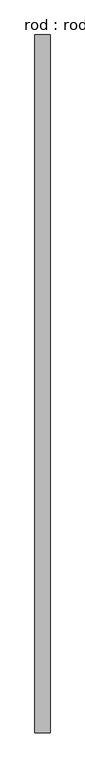
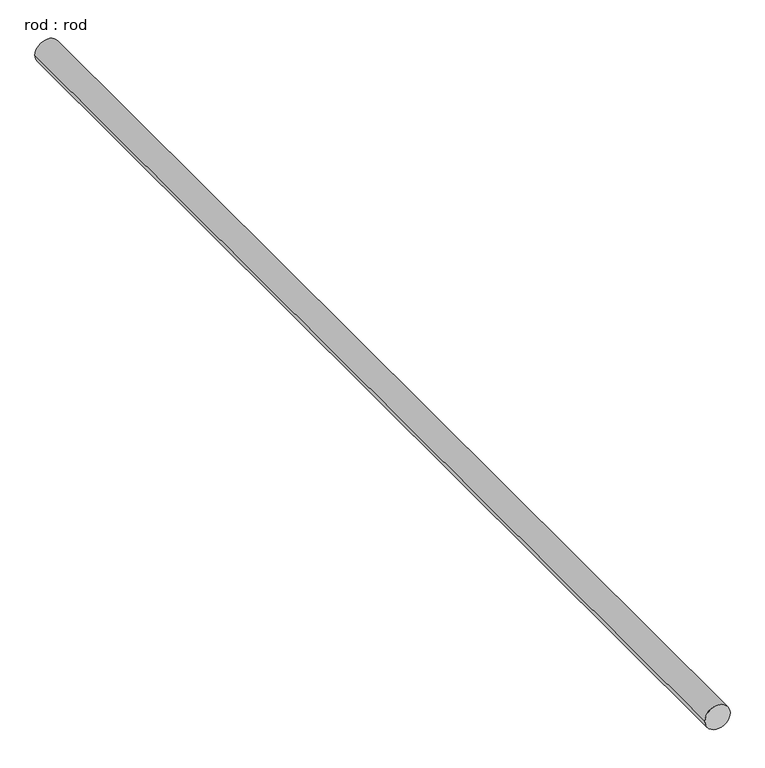
"""IFC4 building model written with IfcOpenShell, lengths in millimetres: proxy geometry, rod : rod."""

import ifcopenshell
import ifcopenshell.guid

model = None  # the IFC model being written
_history = None  # IfcOwnerHistory: only IFC2X3 demands one
_inside = {}  # id of a spatial element -> (the spatial element, [elements in it])
_under = {}  # id of a project, library or spatial element -> (it, [spatial elements below it])
_declared = {}  # id of a project -> (the project, [libraries it declares])
_typed = {}  # id of a type object -> (the type object, [elements of that type])
_made_of = {}  # id of a material, layer set ... -> (it, [elements and type objects made of it])


def new_model(schema):
    """Start an empty IFC model of exactly this schema.

    Asked for "IFC4X3", IfcOpenShell would pick the latest addendum, in which some entities
    have other attributes; the version numbers below select the first issue.
    IFC2X3 requires an IfcOwnerHistory on every rooted entity: one is made here for all.
    """
    global model, _history
    if schema == "IFC4X3":
        model = ifcopenshell.file(schema_version=(4, 3, 0, 0))
    else:
        model = ifcopenshell.file(schema=schema)
    _inside.clear()
    _under.clear()
    _declared.clear()
    _typed.clear()
    _made_of.clear()
    _history = None
    if model.schema == "IFC2X3":
        org = make("IfcOrganization", Name="unknown")
        user = make(
            "IfcPersonAndOrganization",
            ThePerson=make("IfcPerson", FamilyName="unknown"),
            TheOrganization=org,
        )
        app = make(
            "IfcApplication",
            ApplicationDeveloper=org,
            Version="unknown",
            ApplicationFullName="unknown",
            ApplicationIdentifier="unknown",
        )
        _history = make(
            "IfcOwnerHistory",
            OwningUser=user,
            OwningApplication=app,
            ChangeAction="ADDED",
            CreationDate=0,
        )
    return model


def make(cls, **values):
    """One entity of the class cls with the attributes given. An attribute that is None is left unset."""
    return model.create_entity(
        cls, **{name: value for name, value in values.items() if value is not None}
    )


def rooted(cls, **values):
    """An entity with a GlobalId (a new one), such as an element, a storey or a relation."""
    return make(cls, GlobalId=ifcopenshell.guid.new(), OwnerHistory=_history, **values)


def si_unit(unit_type, name, prefix=None):
    """IfcSIUnit, for example si_unit("LENGTHUNIT", "METRE", prefix="MILLI")."""
    return make("IfcSIUnit", UnitType=unit_type, Prefix=prefix, Name=name)


def assignment(units):
    """IfcUnitAssignment: the units of a project."""
    return None if units is None else make("IfcUnitAssignment", Units=units)


def point(xyz):
    """IfcCartesianPoint."""
    return None if xyz is None else make("IfcCartesianPoint", Coordinates=xyz)


def direction(xyz):
    """IfcDirection."""
    return None if xyz is None else make("IfcDirection", DirectionRatios=xyz)


def frame(location, z_axis=None, x_axis=None):
    """IfcAxis2Placement3D, a coordinate frame: its origin and axes. An axis left out is left unset."""
    return make(
        "IfcAxis2Placement3D",
        Location=point(location),
        Axis=direction(z_axis),
        RefDirection=direction(x_axis),
    )


def frame_2d(location, x_axis=None):
    """IfcAxis2Placement2D, a coordinate frame in the plane: its origin and x axis."""
    return make(
        "IfcAxis2Placement2D", Location=point(location), RefDirection=direction(x_axis)
    )


def origin():
    """The frame at (0, 0, 0) with its axes left unset."""
    return frame((0.0, 0.0, 0.0))


def place(relative_to, where):
    """IfcLocalPlacement: puts the frame where relative to a parent placement (None: the world)."""
    return make(
        "IfcLocalPlacement", PlacementRelTo=relative_to, RelativePlacement=where
    )


def context(
    kind, dimensions, precision=None, world=None, true_north=None, identifier=None
):
    """IfcGeometricRepresentationContext, for example the 3D "Model" context."""
    return make(
        "IfcGeometricRepresentationContext",
        ContextIdentifier=identifier,
        ContextType=kind,
        CoordinateSpaceDimension=dimensions,
        Precision=precision,
        WorldCoordinateSystem=world,
        TrueNorth=true_north,
    )


def project(units=None, contexts=None):
    """IfcProject with its units and contexts."""
    return rooted(
        "IfcProject",
        Name="project",
        RepresentationContexts=contexts,
        UnitsInContext=assignment(units),
    )


def spatial(cls, under=None, at=None, **own):
    """A site, building, storey or space (cls), placed at a placement, below another one or the project."""
    s = rooted(cls, ObjectPlacement=at, **own)
    if under is not None:
        _under.setdefault(under.id(), (under, []))[1].append(s)
    return s


def circle_curve(where, radius):
    """IfcCircle in the frame where."""
    return make("IfcCircle", Position=where, Radius=radius)


def trimmed(basis, trim1, trim2, sense, master):
    """IfcTrimmedCurve: the piece of a basis curve between two trims."""
    return make(
        "IfcTrimmedCurve",
        BasisCurve=basis,
        Trim1=trim1,
        Trim2=trim2,
        SenseAgreement=sense,
        MasterRepresentation=master,
    )


def segment(curve, same_sense, transition):
    """IfcCompositeCurveSegment."""
    return make(
        "IfcCompositeCurveSegment",
        Transition=transition,
        SameSense=same_sense,
        ParentCurve=curve,
    )


def composite_curve(segments, self_intersect=None):
    """IfcCompositeCurve: segments joined end to end."""
    return make("IfcCompositeCurve", Segments=segments, SelfIntersect=self_intersect)


def outline(outer, holes=None, kind="AREA"):
    """IfcArbitraryClosedProfileDef: a profile drawn as a closed curve; with holes, ...WithVoids."""
    if holes is None:
        return make("IfcArbitraryClosedProfileDef", ProfileType=kind, OuterCurve=outer)
    return make(
        "IfcArbitraryProfileDefWithVoids",
        ProfileType=kind,
        OuterCurve=outer,
        InnerCurves=holes,
    )


def extrude(swept, where, along, depth):
    """IfcExtrudedAreaSolid: the profile swept, set in the frame where, extruded along a direction by depth."""
    return make(
        "IfcExtrudedAreaSolid",
        SweptArea=swept,
        Position=where,
        ExtrudedDirection=direction(along),
        Depth=depth,
    )


def shape(context_of_items, identifier, shape_type, items):
    """IfcShapeRepresentation: the items that make up one representation, for example the "Body"."""
    return make(
        "IfcShapeRepresentation",
        ContextOfItems=context_of_items,
        RepresentationIdentifier=identifier,
        RepresentationType=shape_type,
        Items=items,
    )


def source(mapping_origin, context_of_items, identifier, shape_type, items):
    """IfcRepresentationMap: a shape defined once, which mapped items show again and again."""
    return make(
        "IfcRepresentationMap",
        MappingOrigin=mapping_origin,
        MappedRepresentation=shape(context_of_items, identifier, shape_type, items),
    )


def transform(
    local_origin,
    x_axis=None,
    y_axis=None,
    z_axis=None,
    scale=None,
    scale2=None,
    scale3=None,
    uniform=True,
):
    """IfcCartesianTransformationOperator3D, or its non-uniform kind. x_axis, y_axis, z_axis: its Axis1, 2, 3."""
    if uniform:
        return make(
            "IfcCartesianTransformationOperator3D",
            Axis1=direction(x_axis),
            Axis2=direction(y_axis),
            LocalOrigin=point(local_origin),
            Scale=scale,
            Axis3=direction(z_axis),
        )
    return make(
        "IfcCartesianTransformationOperator3DnonUniform",
        Axis1=direction(x_axis),
        Axis2=direction(y_axis),
        LocalOrigin=point(local_origin),
        Scale=scale,
        Axis3=direction(z_axis),
        Scale2=scale2,
        Scale3=scale3,
    )


def mapped(mapping_source, mapping_target):
    """IfcMappedItem: shows the shape of a source again, moved by a transform."""
    return make(
        "IfcMappedItem", MappingSource=mapping_source, MappingTarget=mapping_target
    )


def made_of(thing, what):
    """Note that an element or type object is made of a material, layer set ...; save() writes the relation."""
    if what is not None:
        _made_of.setdefault(what.id(), (what, []))[1].append(thing)
    return thing


def element(
    cls,
    number,
    at=None,
    inside=None,
    cuts=None,
    type_object=None,
    material=None,
    context=None,
    identifier="Body",
    shape_type=None,
    held_by="IfcProductDefinitionShape",
    body=None,
    shapes=None,
    **own,
):
    """One element of the class cls, such as IfcWall. Its Tag is "e" and its number.

    at: its placement. inside: the storey or other place that contains it. cuts: it is an
    opening in that element (IfcRelVoidsElement). A single representation is given by context,
    identifier, shape_type and body (its items); several are given by shapes. held_by: the class
    of the entity that holds the representations. save() writes the other relations.
    """
    e = rooted(cls, Tag="e%d" % number, ObjectPlacement=at, **own)
    if body is not None:
        shapes = [shape(context, identifier, shape_type, body)]
    if shapes is not None:
        e.Representation = make(held_by, Representations=shapes)
    if inside is not None:
        _inside.setdefault(inside.id(), (inside, []))[1].append(e)
    if cuts is not None:
        rooted(
            "IfcRelVoidsElement", RelatingBuildingElement=cuts, RelatedOpeningElement=e
        )
    if type_object is not None:
        _typed.setdefault(type_object.id(), (type_object, []))[1].append(e)
    return made_of(e, material)


def aggregate(whole, parts):
    """IfcRelAggregates: a whole, such as a stair, and the parts it consists of."""
    return rooted("IfcRelAggregates", RelatingObject=whole, RelatedObjects=parts)


def save(model, path):
    """Write the relations noted so far, then the file.

    IfcRelAggregates (storeys below a building ...), IfcRelContainedInSpatialStructure (elements
    in a storey), IfcRelDefinesByType, IfcRelAssociatesMaterial and IfcRelDeclares: one each for
    every whole, place, type object, material and project.
    """
    for whole, parts in _under.values():
        aggregate(whole, parts)
    for where, things in _inside.values():
        rooted(
            "IfcRelContainedInSpatialStructure",
            RelatedElements=things,
            RelatingStructure=where,
        )
    for kind, things in _typed.values():
        rooted("IfcRelDefinesByType", RelatedObjects=things, RelatingType=kind)
    for what, things in _made_of.values():
        rooted("IfcRelAssociatesMaterial", RelatedObjects=things, RelatingMaterial=what)
    for by, libraries in _declared.values():
        rooted("IfcRelDeclares", RelatingContext=by, RelatedDefinitions=libraries)
    model.write(path)


def rod_rod_3cca063e(model_context):
    return source(origin(), model_context, "Body", "SweptSolid", [
        extrude(outline(composite_curve([segment(trimmed(circle_curve(frame_2d((0.0108462, 0.0)), 200.0), [point((0.0108462, 200.0))], [point((0.0108462, -200.0))], False, "CARTESIAN"), True, "CONTINUOUS"), segment(trimmed(circle_curve(frame_2d((0.0108462, 0.0)), 200.0), [point((0.0108462, -200.0))], [point((0.0108462, 200.0))], False, "CARTESIAN"), True, "CONTINUOUS")], self_intersect=False)), frame((0.0, -5134.9499561, 0.0), z_axis=(0.0, 1.0, 0.0), x_axis=(0.0, 0.0, 1.0)), (0.0, 0.0, 1.0), 18455.3571429),
    ])


if __name__ == "__main__":
    model = new_model("IFC4")
    model_context = context("Model", 3, world=origin())
    ifc_project = project(units=[si_unit("LENGTHUNIT", "METRE", prefix="MILLI")], contexts=[model_context])
    site = spatial("IfcSite", under=ifc_project)
    building = spatial("IfcBuilding", under=site)
    placement = place(None, origin())
    rod_rod_shape = rod_rod_3cca063e(model_context)
    element("IfcBuildingElementProxy", 1, Name="rod : rod", ObjectType="rod : rod", at=placement, inside=building, context=model_context, shape_type="MappedRepresentation", body=[
        mapped(rod_rod_shape, transform((0.0, 0.0, 0.0), x_axis=(1.0, 0.0, 0.0), y_axis=(0.0, 1.0, 0.0), z_axis=(0.0, 0.0, 1.0))),
    ])
    save(model, "model.ifc")

# Revit data of these elements
# Type "rod : rod"
#   Default Elevation = 0
